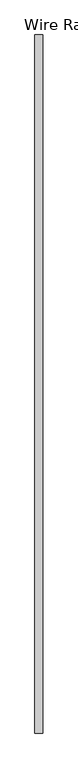
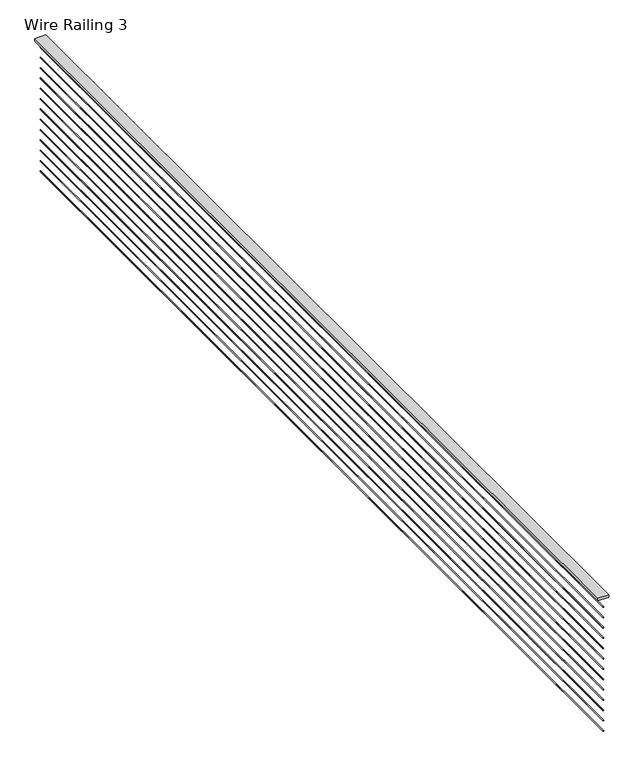
"""IFC4 building model written with IfcOpenShell, lengths in millimetres: railing geometry, Wire Railing 3."""

import ifcopenshell
import ifcopenshell.guid

model = None  # the IFC model being written
_history = None  # IfcOwnerHistory: only IFC2X3 demands one
_inside = {}  # id of a spatial element -> (the spatial element, [elements in it])
_under = {}  # id of a project, library or spatial element -> (it, [spatial elements below it])
_declared = {}  # id of a project -> (the project, [libraries it declares])
_typed = {}  # id of a type object -> (the type object, [elements of that type])
_made_of = {}  # id of a material, layer set ... -> (it, [elements and type objects made of it])


def new_model(schema):
    """Start an empty IFC model of exactly this schema.

    Asked for "IFC4X3", IfcOpenShell would pick the latest addendum, in which some entities
    have other attributes; the version numbers below select the first issue.
    IFC2X3 requires an IfcOwnerHistory on every rooted entity: one is made here for all.
    """
    global model, _history
    if schema == "IFC4X3":
        model = ifcopenshell.file(schema_version=(4, 3, 0, 0))
    else:
        model = ifcopenshell.file(schema=schema)
    _inside.clear()
    _under.clear()
    _declared.clear()
    _typed.clear()
    _made_of.clear()
    _history = None
    if model.schema == "IFC2X3":
        org = make("IfcOrganization", Name="unknown")
        user = make(
            "IfcPersonAndOrganization",
            ThePerson=make("IfcPerson", FamilyName="unknown"),
            TheOrganization=org,
        )
        app = make(
            "IfcApplication",
            ApplicationDeveloper=org,
            Version="unknown",
            ApplicationFullName="unknown",
            ApplicationIdentifier="unknown",
        )
        _history = make(
            "IfcOwnerHistory",
            OwningUser=user,
            OwningApplication=app,
            ChangeAction="ADDED",
            CreationDate=0,
        )
    return model


def make(cls, **values):
    """One entity of the class cls with the attributes given. An attribute that is None is left unset."""
    return model.create_entity(
        cls, **{name: value for name, value in values.items() if value is not None}
    )


def rooted(cls, **values):
    """An entity with a GlobalId (a new one), such as an element, a storey or a relation."""
    return make(cls, GlobalId=ifcopenshell.guid.new(), OwnerHistory=_history, **values)


def si_unit(unit_type, name, prefix=None):
    """IfcSIUnit, for example si_unit("LENGTHUNIT", "METRE", prefix="MILLI")."""
    return make("IfcSIUnit", UnitType=unit_type, Prefix=prefix, Name=name)


def assignment(units):
    """IfcUnitAssignment: the units of a project."""
    return None if units is None else make("IfcUnitAssignment", Units=units)


def point(xyz):
    """IfcCartesianPoint."""
    return None if xyz is None else make("IfcCartesianPoint", Coordinates=xyz)


def direction(xyz):
    """IfcDirection."""
    return None if xyz is None else make("IfcDirection", DirectionRatios=xyz)


def frame(location, z_axis=None, x_axis=None):
    """IfcAxis2Placement3D, a coordinate frame: its origin and axes. An axis left out is left unset."""
    return make(
        "IfcAxis2Placement3D",
        Location=point(location),
        Axis=direction(z_axis),
        RefDirection=direction(x_axis),
    )


def frame_2d(location, x_axis=None):
    """IfcAxis2Placement2D, a coordinate frame in the plane: its origin and x axis."""
    return make(
        "IfcAxis2Placement2D", Location=point(location), RefDirection=direction(x_axis)
    )


def origin():
    """The frame at (0, 0, 0) with its axes left unset."""
    return frame((0.0, 0.0, 0.0))


def place(relative_to, where):
    """IfcLocalPlacement: puts the frame where relative to a parent placement (None: the world)."""
    return make(
        "IfcLocalPlacement", PlacementRelTo=relative_to, RelativePlacement=where
    )


def context(
    kind, dimensions, precision=None, world=None, true_north=None, identifier=None
):
    """IfcGeometricRepresentationContext, for example the 3D "Model" context."""
    return make(
        "IfcGeometricRepresentationContext",
        ContextIdentifier=identifier,
        ContextType=kind,
        CoordinateSpaceDimension=dimensions,
        Precision=precision,
        WorldCoordinateSystem=world,
        TrueNorth=true_north,
    )


def project(units=None, contexts=None):
    """IfcProject with its units and contexts."""
    return rooted(
        "IfcProject",
        Name="project",
        RepresentationContexts=contexts,
        UnitsInContext=assignment(units),
    )


def spatial(cls, under=None, at=None, **own):
    """A site, building, storey or space (cls), placed at a placement, below another one or the project."""
    s = rooted(cls, ObjectPlacement=at, **own)
    if under is not None:
        _under.setdefault(under.id(), (under, []))[1].append(s)
    return s


def polyline(points):
    """IfcPolyline through the points."""
    return make("IfcPolyline", Points=[point(p) for p in points])


def circle_curve(where, radius):
    """IfcCircle in the frame where."""
    return make("IfcCircle", Position=where, Radius=radius)


def trimmed(basis, trim1, trim2, sense, master):
    """IfcTrimmedCurve: the piece of a basis curve between two trims."""
    return make(
        "IfcTrimmedCurve",
        BasisCurve=basis,
        Trim1=trim1,
        Trim2=trim2,
        SenseAgreement=sense,
        MasterRepresentation=master,
    )


def segment(curve, same_sense, transition):
    """IfcCompositeCurveSegment."""
    return make(
        "IfcCompositeCurveSegment",
        Transition=transition,
        SameSense=same_sense,
        ParentCurve=curve,
    )


def composite_curve(segments, self_intersect=None):
    """IfcCompositeCurve: segments joined end to end."""
    return make("IfcCompositeCurve", Segments=segments, SelfIntersect=self_intersect)


def outline(outer, holes=None, kind="AREA"):
    """IfcArbitraryClosedProfileDef: a profile drawn as a closed curve; with holes, ...WithVoids."""
    if holes is None:
        return make("IfcArbitraryClosedProfileDef", ProfileType=kind, OuterCurve=outer)
    return make(
        "IfcArbitraryProfileDefWithVoids",
        ProfileType=kind,
        OuterCurve=outer,
        InnerCurves=holes,
    )


def extrude(swept, where, along, depth):
    """IfcExtrudedAreaSolid: the profile swept, set in the frame where, extruded along a direction by depth."""
    return make(
        "IfcExtrudedAreaSolid",
        SweptArea=swept,
        Position=where,
        ExtrudedDirection=direction(along),
        Depth=depth,
    )


def shape(context_of_items, identifier, shape_type, items):
    """IfcShapeRepresentation: the items that make up one representation, for example the "Body"."""
    return make(
        "IfcShapeRepresentation",
        ContextOfItems=context_of_items,
        RepresentationIdentifier=identifier,
        RepresentationType=shape_type,
        Items=items,
    )


def source(mapping_origin, context_of_items, identifier, shape_type, items):
    """IfcRepresentationMap: a shape defined once, which mapped items show again and again."""
    return make(
        "IfcRepresentationMap",
        MappingOrigin=mapping_origin,
        MappedRepresentation=shape(context_of_items, identifier, shape_type, items),
    )


def transform(
    local_origin,
    x_axis=None,
    y_axis=None,
    z_axis=None,
    scale=None,
    scale2=None,
    scale3=None,
    uniform=True,
):
    """IfcCartesianTransformationOperator3D, or its non-uniform kind. x_axis, y_axis, z_axis: its Axis1, 2, 3."""
    if uniform:
        return make(
            "IfcCartesianTransformationOperator3D",
            Axis1=direction(x_axis),
            Axis2=direction(y_axis),
            LocalOrigin=point(local_origin),
            Scale=scale,
            Axis3=direction(z_axis),
        )
    return make(
        "IfcCartesianTransformationOperator3DnonUniform",
        Axis1=direction(x_axis),
        Axis2=direction(y_axis),
        LocalOrigin=point(local_origin),
        Scale=scale,
        Axis3=direction(z_axis),
        Scale2=scale2,
        Scale3=scale3,
    )


def mapped(mapping_source, mapping_target):
    """IfcMappedItem: shows the shape of a source again, moved by a transform."""
    return make(
        "IfcMappedItem", MappingSource=mapping_source, MappingTarget=mapping_target
    )


def made_of(thing, what):
    """Note that an element or type object is made of a material, layer set ...; save() writes the relation."""
    if what is not None:
        _made_of.setdefault(what.id(), (what, []))[1].append(thing)
    return thing


def element(
    cls,
    number,
    at=None,
    inside=None,
    cuts=None,
    type_object=None,
    material=None,
    context=None,
    identifier="Body",
    shape_type=None,
    held_by="IfcProductDefinitionShape",
    body=None,
    shapes=None,
    **own,
):
    """One element of the class cls, such as IfcWall. Its Tag is "e" and its number.

    at: its placement. inside: the storey or other place that contains it. cuts: it is an
    opening in that element (IfcRelVoidsElement). A single representation is given by context,
    identifier, shape_type and body (its items); several are given by shapes. held_by: the class
    of the entity that holds the representations. save() writes the other relations.
    """
    e = rooted(cls, Tag="e%d" % number, ObjectPlacement=at, **own)
    if body is not None:
        shapes = [shape(context, identifier, shape_type, body)]
    if shapes is not None:
        e.Representation = make(held_by, Representations=shapes)
    if inside is not None:
        _inside.setdefault(inside.id(), (inside, []))[1].append(e)
    if cuts is not None:
        rooted(
            "IfcRelVoidsElement", RelatingBuildingElement=cuts, RelatedOpeningElement=e
        )
    if type_object is not None:
        _typed.setdefault(type_object.id(), (type_object, []))[1].append(e)
    return made_of(e, material)


def aggregate(whole, parts):
    """IfcRelAggregates: a whole, such as a stair, and the parts it consists of."""
    return rooted("IfcRelAggregates", RelatingObject=whole, RelatedObjects=parts)


def save(model, path):
    """Write the relations noted so far, then the file.

    IfcRelAggregates (storeys below a building ...), IfcRelContainedInSpatialStructure (elements
    in a storey), IfcRelDefinesByType, IfcRelAssociatesMaterial and IfcRelDeclares: one each for
    every whole, place, type object, material and project.
    """
    for whole, parts in _under.values():
        aggregate(whole, parts)
    for where, things in _inside.values():
        rooted(
            "IfcRelContainedInSpatialStructure",
            RelatedElements=things,
            RelatingStructure=where,
        )
    for kind, things in _typed.values():
        rooted("IfcRelDefinesByType", RelatedObjects=things, RelatingType=kind)
    for what, things in _made_of.values():
        rooted("IfcRelAssociatesMaterial", RelatedObjects=things, RelatingMaterial=what)
    for by, libraries in _declared.values():
        rooted("IfcRelDeclares", RelatingContext=by, RelatedDefinitions=libraries)
    model.write(path)


def wire_railing_3_fa1d4893(model_context):
    return source(origin(), model_context, "Body", "SweptSolid", [
        extrude(outline(polyline([(22206.7370052, -2519.6884634), (22130.5370052, -2519.6884634), (22130.5370052, 4293.1885346), (22206.7370052, 4293.1885346), (22206.7370052, -2519.6884634)])), frame((0.0, 0.0, 3740.15), z_axis=(0.0, 0.0, 1.0), x_axis=(1.0, 0.0, 0.0)), (0.0, 0.0, 1.0), 19.05),
        extrude(outline(composite_curve([segment(trimmed(circle_curve(frame_2d((3680.61875, 22168.6370052)), 2.38125), [point((3680.61875, 22166.2557552))], [point((3680.61875, 22171.0182552))], False, "CARTESIAN"), True, "CONTINUOUS"), segment(trimmed(circle_curve(frame_2d((3680.61875, 22168.6370052)), 2.38125), [point((3680.61875, 22171.0182552))], [point((3680.61875, 22166.2557552))], False, "CARTESIAN"), True, "CONTINUOUS")], self_intersect=False)), frame((0.0, -2519.6884634, 0.0), z_axis=(0.0, 1.0, 0.0), x_axis=(0.0, 0.0, 1.0)), (0.0, 0.0, 1.0), 6812.876998),
        extrude(outline(composite_curve([segment(trimmed(circle_curve(frame_2d((3604.41875, 22168.6370052)), 2.38125), [point((3604.41875, 22166.2557552))], [point((3604.41875, 22171.0182552))], False, "CARTESIAN"), True, "CONTINUOUS"), segment(trimmed(circle_curve(frame_2d((3604.41875, 22168.6370052)), 2.38125), [point((3604.41875, 22171.0182552))], [point((3604.41875, 22166.2557552))], False, "CARTESIAN"), True, "CONTINUOUS")], self_intersect=False)), frame((0.0, -2519.6884634, 0.0), z_axis=(0.0, 1.0, 0.0), x_axis=(0.0, 0.0, 1.0)), (0.0, 0.0, 1.0), 6812.876998),
        extrude(outline(composite_curve([segment(trimmed(circle_curve(frame_2d((3528.21875, 22168.6370052)), 2.38125), [point((3528.21875, 22166.2557552))], [point((3528.21875, 22171.0182552))], False, "CARTESIAN"), True, "CONTINUOUS"), segment(trimmed(circle_curve(frame_2d((3528.21875, 22168.6370052)), 2.38125), [point((3528.21875, 22171.0182552))], [point((3528.21875, 22166.2557552))], False, "CARTESIAN"), True, "CONTINUOUS")], self_intersect=False)), frame((0.0, -2519.6884634, 0.0), z_axis=(0.0, 1.0, 0.0), x_axis=(0.0, 0.0, 1.0)), (0.0, 0.0, 1.0), 6812.876998),
        extrude(outline(composite_curve([segment(trimmed(circle_curve(frame_2d((3452.01875, 22168.6370052)), 2.38125), [point((3452.01875, 22166.2557552))], [point((3452.01875, 22171.0182552))], False, "CARTESIAN"), True, "CONTINUOUS"), segment(trimmed(circle_curve(frame_2d((3452.01875, 22168.6370052)), 2.38125), [point((3452.01875, 22171.0182552))], [point((3452.01875, 22166.2557552))], False, "CARTESIAN"), True, "CONTINUOUS")], self_intersect=False)), frame((0.0, -2519.6884634, 0.0), z_axis=(0.0, 1.0, 0.0), x_axis=(0.0, 0.0, 1.0)), (0.0, 0.0, 1.0), 6812.876998),
        extrude(outline(composite_curve([segment(trimmed(circle_curve(frame_2d((3375.81875, 22168.6370052)), 2.38125), [point((3375.81875, 22166.2557552))], [point((3375.81875, 22171.0182552))], False, "CARTESIAN"), True, "CONTINUOUS"), segment(trimmed(circle_curve(frame_2d((3375.81875, 22168.6370052)), 2.38125), [point((3375.81875, 22171.0182552))], [point((3375.81875, 22166.2557552))], False, "CARTESIAN"), True, "CONTINUOUS")], self_intersect=False)), frame((0.0, -2519.6884634, 0.0), z_axis=(0.0, 1.0, 0.0), x_axis=(0.0, 0.0, 1.0)), (0.0, 0.0, 1.0), 6812.876998),
        extrude(outline(composite_curve([segment(trimmed(circle_curve(frame_2d((3299.61875, 22168.6370052)), 2.38125), [point((3299.61875, 22166.2557552))], [point((3299.61875, 22171.0182552))], False, "CARTESIAN"), True, "CONTINUOUS"), segment(trimmed(circle_curve(frame_2d((3299.61875, 22168.6370052)), 2.38125), [point((3299.61875, 22171.0182552))], [point((3299.61875, 22166.2557552))], False, "CARTESIAN"), True, "CONTINUOUS")], self_intersect=False)), frame((0.0, -2519.6884634, 0.0), z_axis=(0.0, 1.0, 0.0), x_axis=(0.0, 0.0, 1.0)), (0.0, 0.0, 1.0), 6812.876998),
        extrude(outline(composite_curve([segment(trimmed(circle_curve(frame_2d((3223.41875, 22168.6370052)), 2.38125), [point((3223.41875, 22166.2557552))], [point((3223.41875, 22171.0182552))], False, "CARTESIAN"), True, "CONTINUOUS"), segment(trimmed(circle_curve(frame_2d((3223.41875, 22168.6370052)), 2.38125), [point((3223.41875, 22171.0182552))], [point((3223.41875, 22166.2557552))], False, "CARTESIAN"), True, "CONTINUOUS")], self_intersect=False)), frame((0.0, -2519.6884634, 0.0), z_axis=(0.0, 1.0, 0.0), x_axis=(0.0, 0.0, 1.0)), (0.0, 0.0, 1.0), 6812.876998),
        extrude(outline(composite_curve([segment(trimmed(circle_curve(frame_2d((3147.21875, 22168.6370052)), 2.38125), [point((3147.21875, 22166.2557552))], [point((3147.21875, 22171.0182552))], False, "CARTESIAN"), True, "CONTINUOUS"), segment(trimmed(circle_curve(frame_2d((3147.21875, 22168.6370052)), 2.38125), [point((3147.21875, 22171.0182552))], [point((3147.21875, 22166.2557552))], False, "CARTESIAN"), True, "CONTINUOUS")], self_intersect=False)), frame((0.0, -2519.6884634, 0.0), z_axis=(0.0, 1.0, 0.0), x_axis=(0.0, 0.0, 1.0)), (0.0, 0.0, 1.0), 6812.876998),
        extrude(outline(composite_curve([segment(trimmed(circle_curve(frame_2d((3071.01875, 22168.6370052)), 2.38125), [point((3071.01875, 22166.2557552))], [point((3071.01875, 22171.0182552))], False, "CARTESIAN"), True, "CONTINUOUS"), segment(trimmed(circle_curve(frame_2d((3071.01875, 22168.6370052)), 2.38125), [point((3071.01875, 22171.0182552))], [point((3071.01875, 22166.2557552))], False, "CARTESIAN"), True, "CONTINUOUS")], self_intersect=False)), frame((0.0, -2519.6884634, 0.0), z_axis=(0.0, 1.0, 0.0), x_axis=(0.0, 0.0, 1.0)), (0.0, 0.0, 1.0), 6812.876998),
        extrude(outline(composite_curve([segment(trimmed(circle_curve(frame_2d((2994.81875, 22168.6370052)), 2.38125), [point((2994.81875, 22166.2557552))], [point((2994.81875, 22171.0182552))], False, "CARTESIAN"), True, "CONTINUOUS"), segment(trimmed(circle_curve(frame_2d((2994.81875, 22168.6370052)), 2.38125), [point((2994.81875, 22171.0182552))], [point((2994.81875, 22166.2557552))], False, "CARTESIAN"), True, "CONTINUOUS")], self_intersect=False)), frame((0.0, -2519.6884634, 0.0), z_axis=(0.0, 1.0, 0.0), x_axis=(0.0, 0.0, 1.0)), (0.0, 0.0, 1.0), 6812.876998),
        extrude(outline(composite_curve([segment(trimmed(circle_curve(frame_2d((2918.61875, 22168.6370052)), 2.38125), [point((2918.61875, 22166.2557552))], [point((2918.61875, 22171.0182552))], False, "CARTESIAN"), True, "CONTINUOUS"), segment(trimmed(circle_curve(frame_2d((2918.61875, 22168.6370052)), 2.38125), [point((2918.61875, 22171.0182552))], [point((2918.61875, 22166.2557552))], False, "CARTESIAN"), True, "CONTINUOUS")], self_intersect=False)), frame((0.0, -2519.6884634, 0.0), z_axis=(0.0, 1.0, 0.0), x_axis=(0.0, 0.0, 1.0)), (0.0, 0.0, 1.0), 6812.876998),
        extrude(outline(composite_curve([segment(trimmed(circle_curve(frame_2d((2842.41875, 22168.6370052)), 2.38125), [point((2842.41875, 22166.2557552))], [point((2842.41875, 22171.0182552))], False, "CARTESIAN"), True, "CONTINUOUS"), segment(trimmed(circle_curve(frame_2d((2842.41875, 22168.6370052)), 2.38125), [point((2842.41875, 22171.0182552))], [point((2842.41875, 22166.2557552))], False, "CARTESIAN"), True, "CONTINUOUS")], self_intersect=False)), frame((0.0, -2519.6884634, 0.0), z_axis=(0.0, 1.0, 0.0), x_axis=(0.0, 0.0, 1.0)), (0.0, 0.0, 1.0), 6812.876998),
        extrude(outline(composite_curve([segment(trimmed(circle_curve(frame_2d((2766.21875, 22168.6370052)), 2.38125), [point((2766.21875, 22166.2557552))], [point((2766.21875, 22171.0182552))], False, "CARTESIAN"), True, "CONTINUOUS"), segment(trimmed(circle_curve(frame_2d((2766.21875, 22168.6370052)), 2.38125), [point((2766.21875, 22171.0182552))], [point((2766.21875, 22166.2557552))], False, "CARTESIAN"), True, "CONTINUOUS")], self_intersect=False)), frame((0.0, -2519.6884634, 0.0), z_axis=(0.0, 1.0, 0.0), x_axis=(0.0, 0.0, 1.0)), (0.0, 0.0, 1.0), 6812.876998),
    ])


if __name__ == "__main__":
    model = new_model("IFC4")
    model_context = context("Model", 3, world=origin())
    ifc_project = project(units=[si_unit("LENGTHUNIT", "METRE", prefix="MILLI")], contexts=[model_context])
    site = spatial("IfcSite", under=ifc_project)
    building = spatial("IfcBuilding", under=site)
    placement = place(None, origin())
    wire_railing_3_shape = wire_railing_3_fa1d4893(model_context)
    element("IfcRailing", 1, ObjectType="Wire Railing 3", at=placement, inside=building, context=model_context, shape_type="MappedRepresentation", body=[
        mapped(wire_railing_3_shape, transform((0.0, 0.0, 0.0), x_axis=(1.0, 0.0, 0.0), y_axis=(0.0, 1.0, 0.0), z_axis=(0.0, 0.0, 1.0))),
    ])
    save(model, "model.ifc")

# Revit data of these elements
# Element 1 (IfcRailing, "Wire Railing 3")
#   Materials on its faces: "WIRE RAILING (3\" O.C.)", "ALUM. PLATE TOP RAIL"
# Materials
#   "WIRE RAILING (3\" O.C.)": class "Metal", colour RGB 244 244 244, transparency 0, Manufacturer = "Kawneer", URL = "http://www.kawneer.com/kawneer/north_america/en/home.asp", Cost = 0
#   "ALUM. PLATE TOP RAIL": class "Metal", colour RGB 244 244 244, transparency 0, Manufacturer = "Kawneer", URL = "http://www.kawneer.com/kawneer/north_america/en/home.asp", Cost = 0
